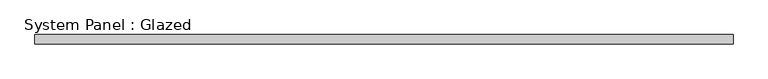
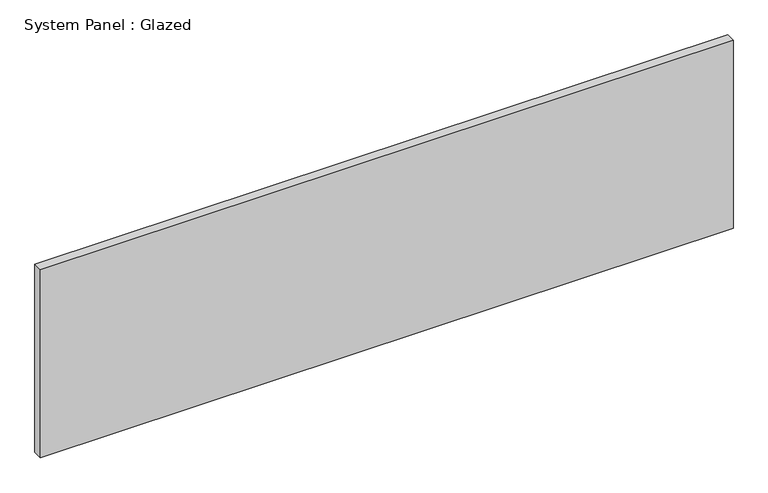
"""IFC4 building model written with IfcOpenShell, lengths in millimetres: plate geometry, System Panel : Glazed."""

from ifc_helpers import new_model, si_unit, origin, origin_with_axes, place, context, project, spatial, polyline, outline, extrude, source, transform, mapped, element, save


def system_panel_glazed_da03e73d(model_context):
    return source(origin(), model_context, "Body", "SweptSolid", [
        extrude(outline(polyline([(915.0000002, 24.5), (-915.0000002, 24.5), (-915.0000002, 49.5), (915.0000002, 49.5), (915.0000002, 24.5)])), origin_with_axes(), (0.0, 0.0, 1.0), 525.0),
    ])


if __name__ == "__main__":
    model = new_model("IFC4")
    model_context = context("Model", 3, world=origin())
    ifc_project = project(units=[si_unit("LENGTHUNIT", "METRE", prefix="MILLI")], contexts=[model_context])
    site = spatial("IfcSite", under=ifc_project)
    building = spatial("IfcBuilding", under=site)
    placement = place(None, origin())
    system_panel_glazed_shape = system_panel_glazed_da03e73d(model_context)
    element("IfcPlate", 1, ObjectType="System Panel : Glazed", at=placement, inside=building, context=model_context, shape_type="MappedRepresentation", body=[
        mapped(system_panel_glazed_shape, transform((0.0, 0.0, 0.0), x_axis=(1.0, 0.0, 0.0), y_axis=(0.0, 1.0, 0.0), z_axis=(0.0, 0.0, 1.0))),
    ])
    save(model, "model.ifc")

# Revit data of these elements
# Element 1 (IfcPlate, "System Panel : Glazed")
#   Materials on its faces: "Glass"
# Materials
#   "Glass": class "Glass", colour RGB 218 227 224, transparency 0.85, Description = "Soda Lime Glass", Cost = 0
